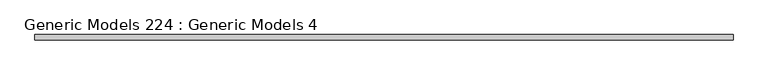
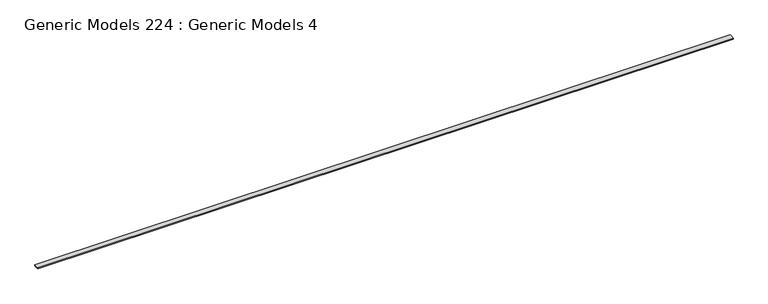
"""IFC4 building model written with IfcOpenShell, lengths in millimetres: proxy geometry, Generic Models 224 : Generic Models 4."""

from ifc_helpers import new_model, si_unit, frame, origin, place, context, project, spatial, polyline, outline, extrude, source, transform, mapped, element, save


def generic_models_224_generic_models_4_4e20d8a3(model_context):
    return source(origin(), model_context, "Body", "SweptSolid", [
        extrude(outline(polyline([(-29182.8735041, 127104.4735933), (-29322.5735041, 127104.4735933), (-29322.5735041, 127136.7527599), (-29182.8735041, 127142.5735933), (-29182.8735041, 127104.4735933)])), frame((-20795.7733045, 0.0, 0.0), z_axis=(1.0, 0.0, 0.0), x_axis=(0.0, 1.0, 0.0)), (0.0, 0.0, 1.0), 18643.6),
    ])


if __name__ == "__main__":
    model = new_model("IFC4")
    model_context = context("Model", 3, world=origin())
    ifc_project = project(units=[si_unit("LENGTHUNIT", "METRE", prefix="MILLI")], contexts=[model_context])
    site = spatial("IfcSite", under=ifc_project)
    building = spatial("IfcBuilding", under=site)
    placement = place(None, origin())
    generic_models_224_generic_models_4_shape = generic_models_224_generic_models_4_4e20d8a3(model_context)
    element("IfcBuildingElementProxy", 1, Name="Generic Models 224 : Generic Models 4", ObjectType="Generic Models 224 : Generic Models 4", at=placement, inside=building, context=model_context, shape_type="MappedRepresentation", body=[
        mapped(generic_models_224_generic_models_4_shape, transform((0.0, 0.0, 0.0), x_axis=(1.0, 0.0, 0.0), y_axis=(0.0, 1.0, 0.0), z_axis=(0.0, 0.0, 1.0))),
    ])
    save(model, "model.ifc")

# Revit data of these elements
# Element 1 (IfcBuildingElementProxy, "Generic Models 224 : Generic Models 4")
#   Materials on its faces: "_2X BLOCKING AS REQUIRED"
# Materials
#   "_2X BLOCKING AS REQUIRED": class "Generic", colour RGB 177 130 114, transparency 0, Cost = 0
